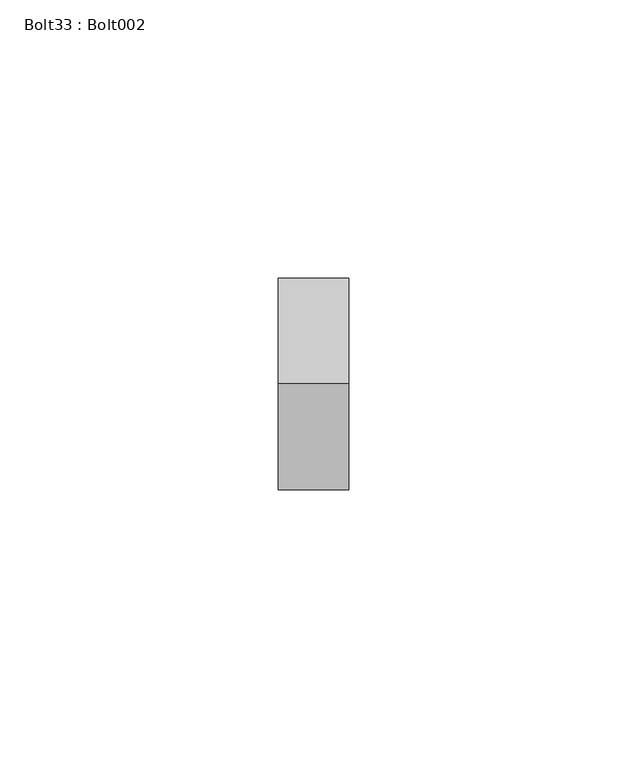
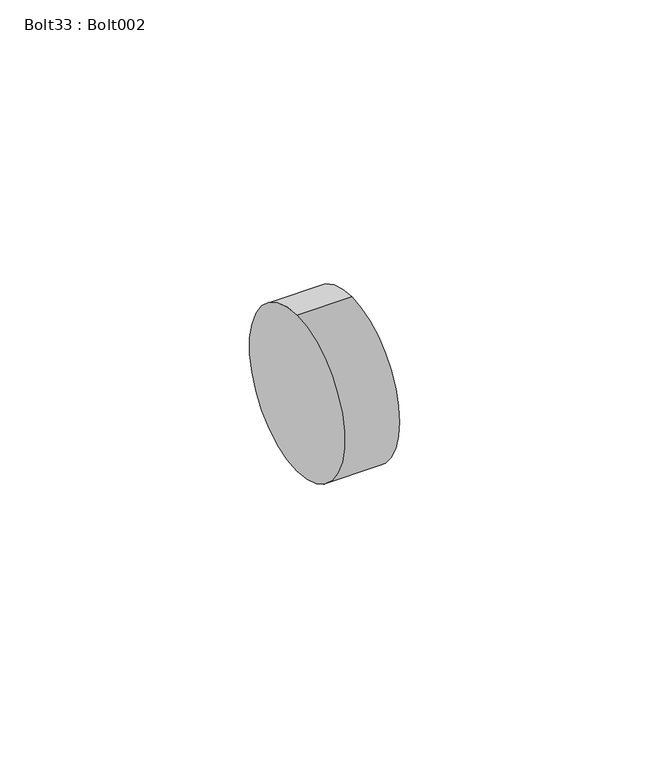
"""IFC4 building model written with IfcOpenShell, lengths in millimetres: proxy geometry, Bolt33 : Bolt002."""

import ifcopenshell
import ifcopenshell.guid

model = None  # the IFC model being written
_history = None  # IfcOwnerHistory: only IFC2X3 demands one
_inside = {}  # id of a spatial element -> (the spatial element, [elements in it])
_under = {}  # id of a project, library or spatial element -> (it, [spatial elements below it])
_declared = {}  # id of a project -> (the project, [libraries it declares])
_typed = {}  # id of a type object -> (the type object, [elements of that type])
_made_of = {}  # id of a material, layer set ... -> (it, [elements and type objects made of it])


def new_model(schema):
    """Start an empty IFC model of exactly this schema.

    Asked for "IFC4X3", IfcOpenShell would pick the latest addendum, in which some entities
    have other attributes; the version numbers below select the first issue.
    IFC2X3 requires an IfcOwnerHistory on every rooted entity: one is made here for all.
    """
    global model, _history
    if schema == "IFC4X3":
        model = ifcopenshell.file(schema_version=(4, 3, 0, 0))
    else:
        model = ifcopenshell.file(schema=schema)
    _inside.clear()
    _under.clear()
    _declared.clear()
    _typed.clear()
    _made_of.clear()
    _history = None
    if model.schema == "IFC2X3":
        org = make("IfcOrganization", Name="unknown")
        user = make(
            "IfcPersonAndOrganization",
            ThePerson=make("IfcPerson", FamilyName="unknown"),
            TheOrganization=org,
        )
        app = make(
            "IfcApplication",
            ApplicationDeveloper=org,
            Version="unknown",
            ApplicationFullName="unknown",
            ApplicationIdentifier="unknown",
        )
        _history = make(
            "IfcOwnerHistory",
            OwningUser=user,
            OwningApplication=app,
            ChangeAction="ADDED",
            CreationDate=0,
        )
    return model


def make(cls, **values):
    """One entity of the class cls with the attributes given. An attribute that is None is left unset."""
    return model.create_entity(
        cls, **{name: value for name, value in values.items() if value is not None}
    )


def rooted(cls, **values):
    """An entity with a GlobalId (a new one), such as an element, a storey or a relation."""
    return make(cls, GlobalId=ifcopenshell.guid.new(), OwnerHistory=_history, **values)


def si_unit(unit_type, name, prefix=None):
    """IfcSIUnit, for example si_unit("LENGTHUNIT", "METRE", prefix="MILLI")."""
    return make("IfcSIUnit", UnitType=unit_type, Prefix=prefix, Name=name)


def assignment(units):
    """IfcUnitAssignment: the units of a project."""
    return None if units is None else make("IfcUnitAssignment", Units=units)


def point(xyz):
    """IfcCartesianPoint."""
    return None if xyz is None else make("IfcCartesianPoint", Coordinates=xyz)


def direction(xyz):
    """IfcDirection."""
    return None if xyz is None else make("IfcDirection", DirectionRatios=xyz)


def frame(location, z_axis=None, x_axis=None):
    """IfcAxis2Placement3D, a coordinate frame: its origin and axes. An axis left out is left unset."""
    return make(
        "IfcAxis2Placement3D",
        Location=point(location),
        Axis=direction(z_axis),
        RefDirection=direction(x_axis),
    )


def frame_2d(location, x_axis=None):
    """IfcAxis2Placement2D, a coordinate frame in the plane: its origin and x axis."""
    return make(
        "IfcAxis2Placement2D", Location=point(location), RefDirection=direction(x_axis)
    )


def origin():
    """The frame at (0, 0, 0) with its axes left unset."""
    return frame((0.0, 0.0, 0.0))


def place(relative_to, where):
    """IfcLocalPlacement: puts the frame where relative to a parent placement (None: the world)."""
    return make(
        "IfcLocalPlacement", PlacementRelTo=relative_to, RelativePlacement=where
    )


def context(
    kind, dimensions, precision=None, world=None, true_north=None, identifier=None
):
    """IfcGeometricRepresentationContext, for example the 3D "Model" context."""
    return make(
        "IfcGeometricRepresentationContext",
        ContextIdentifier=identifier,
        ContextType=kind,
        CoordinateSpaceDimension=dimensions,
        Precision=precision,
        WorldCoordinateSystem=world,
        TrueNorth=true_north,
    )


def project(units=None, contexts=None):
    """IfcProject with its units and contexts."""
    return rooted(
        "IfcProject",
        Name="project",
        RepresentationContexts=contexts,
        UnitsInContext=assignment(units),
    )


def spatial(cls, under=None, at=None, **own):
    """A site, building, storey or space (cls), placed at a placement, below another one or the project."""
    s = rooted(cls, ObjectPlacement=at, **own)
    if under is not None:
        _under.setdefault(under.id(), (under, []))[1].append(s)
    return s


def circle_curve(where, radius):
    """IfcCircle in the frame where."""
    return make("IfcCircle", Position=where, Radius=radius)


def trimmed(basis, trim1, trim2, sense, master):
    """IfcTrimmedCurve: the piece of a basis curve between two trims."""
    return make(
        "IfcTrimmedCurve",
        BasisCurve=basis,
        Trim1=trim1,
        Trim2=trim2,
        SenseAgreement=sense,
        MasterRepresentation=master,
    )


def segment(curve, same_sense, transition):
    """IfcCompositeCurveSegment."""
    return make(
        "IfcCompositeCurveSegment",
        Transition=transition,
        SameSense=same_sense,
        ParentCurve=curve,
    )


def composite_curve(segments, self_intersect=None):
    """IfcCompositeCurve: segments joined end to end."""
    return make("IfcCompositeCurve", Segments=segments, SelfIntersect=self_intersect)


def outline(outer, holes=None, kind="AREA"):
    """IfcArbitraryClosedProfileDef: a profile drawn as a closed curve; with holes, ...WithVoids."""
    if holes is None:
        return make("IfcArbitraryClosedProfileDef", ProfileType=kind, OuterCurve=outer)
    return make(
        "IfcArbitraryProfileDefWithVoids",
        ProfileType=kind,
        OuterCurve=outer,
        InnerCurves=holes,
    )


def extrude(swept, where, along, depth):
    """IfcExtrudedAreaSolid: the profile swept, set in the frame where, extruded along a direction by depth."""
    return make(
        "IfcExtrudedAreaSolid",
        SweptArea=swept,
        Position=where,
        ExtrudedDirection=direction(along),
        Depth=depth,
    )


def shape(context_of_items, identifier, shape_type, items):
    """IfcShapeRepresentation: the items that make up one representation, for example the "Body"."""
    return make(
        "IfcShapeRepresentation",
        ContextOfItems=context_of_items,
        RepresentationIdentifier=identifier,
        RepresentationType=shape_type,
        Items=items,
    )


def source(mapping_origin, context_of_items, identifier, shape_type, items):
    """IfcRepresentationMap: a shape defined once, which mapped items show again and again."""
    return make(
        "IfcRepresentationMap",
        MappingOrigin=mapping_origin,
        MappedRepresentation=shape(context_of_items, identifier, shape_type, items),
    )


def transform(
    local_origin,
    x_axis=None,
    y_axis=None,
    z_axis=None,
    scale=None,
    scale2=None,
    scale3=None,
    uniform=True,
):
    """IfcCartesianTransformationOperator3D, or its non-uniform kind. x_axis, y_axis, z_axis: its Axis1, 2, 3."""
    if uniform:
        return make(
            "IfcCartesianTransformationOperator3D",
            Axis1=direction(x_axis),
            Axis2=direction(y_axis),
            LocalOrigin=point(local_origin),
            Scale=scale,
            Axis3=direction(z_axis),
        )
    return make(
        "IfcCartesianTransformationOperator3DnonUniform",
        Axis1=direction(x_axis),
        Axis2=direction(y_axis),
        LocalOrigin=point(local_origin),
        Scale=scale,
        Axis3=direction(z_axis),
        Scale2=scale2,
        Scale3=scale3,
    )


def mapped(mapping_source, mapping_target):
    """IfcMappedItem: shows the shape of a source again, moved by a transform."""
    return make(
        "IfcMappedItem", MappingSource=mapping_source, MappingTarget=mapping_target
    )


def made_of(thing, what):
    """Note that an element or type object is made of a material, layer set ...; save() writes the relation."""
    if what is not None:
        _made_of.setdefault(what.id(), (what, []))[1].append(thing)
    return thing


def element(
    cls,
    number,
    at=None,
    inside=None,
    cuts=None,
    type_object=None,
    material=None,
    context=None,
    identifier="Body",
    shape_type=None,
    held_by="IfcProductDefinitionShape",
    body=None,
    shapes=None,
    **own,
):
    """One element of the class cls, such as IfcWall. Its Tag is "e" and its number.

    at: its placement. inside: the storey or other place that contains it. cuts: it is an
    opening in that element (IfcRelVoidsElement). A single representation is given by context,
    identifier, shape_type and body (its items); several are given by shapes. held_by: the class
    of the entity that holds the representations. save() writes the other relations.
    """
    e = rooted(cls, Tag="e%d" % number, ObjectPlacement=at, **own)
    if body is not None:
        shapes = [shape(context, identifier, shape_type, body)]
    if shapes is not None:
        e.Representation = make(held_by, Representations=shapes)
    if inside is not None:
        _inside.setdefault(inside.id(), (inside, []))[1].append(e)
    if cuts is not None:
        rooted(
            "IfcRelVoidsElement", RelatingBuildingElement=cuts, RelatedOpeningElement=e
        )
    if type_object is not None:
        _typed.setdefault(type_object.id(), (type_object, []))[1].append(e)
    return made_of(e, material)


def aggregate(whole, parts):
    """IfcRelAggregates: a whole, such as a stair, and the parts it consists of."""
    return rooted("IfcRelAggregates", RelatingObject=whole, RelatedObjects=parts)


def save(model, path):
    """Write the relations noted so far, then the file.

    IfcRelAggregates (storeys below a building ...), IfcRelContainedInSpatialStructure (elements
    in a storey), IfcRelDefinesByType, IfcRelAssociatesMaterial and IfcRelDeclares: one each for
    every whole, place, type object, material and project.
    """
    for whole, parts in _under.values():
        aggregate(whole, parts)
    for where, things in _inside.values():
        rooted(
            "IfcRelContainedInSpatialStructure",
            RelatedElements=things,
            RelatingStructure=where,
        )
    for kind, things in _typed.values():
        rooted("IfcRelDefinesByType", RelatedObjects=things, RelatingType=kind)
    for what, things in _made_of.values():
        rooted("IfcRelAssociatesMaterial", RelatedObjects=things, RelatingMaterial=what)
    for by, libraries in _declared.values():
        rooted("IfcRelDeclares", RelatingContext=by, RelatedDefinitions=libraries)
    model.write(path)


def bolt33_bolt002_dc929be4(model_context):
    return source(origin(), model_context, "Body", "SweptSolid", [
        extrude(outline(composite_curve([segment(trimmed(circle_curve(frame_2d((1896.5882072, 40070.0545241)), 19.05), [point((1896.5882072, 40051.0045241))], [point((1896.5882072, 40089.1045241))], False, "CARTESIAN"), True, "CONTINUOUS"), segment(trimmed(circle_curve(frame_2d((1896.5882072, 40070.0545241)), 19.05), [point((1896.5882072, 40089.1045241))], [point((1896.5882072, 40051.0045241))], False, "CARTESIAN"), True, "CONTINUOUS")], self_intersect=False)), frame((10268.2640809, 0.0, 0.0), z_axis=(1.0, 0.0, 0.0), x_axis=(0.0, 1.0, 0.0)), (0.0, 0.0, 1.0), 12.7),
    ])


if __name__ == "__main__":
    model = new_model("IFC4")
    model_context = context("Model", 3, world=origin())
    ifc_project = project(units=[si_unit("LENGTHUNIT", "METRE", prefix="MILLI")], contexts=[model_context])
    site = spatial("IfcSite", under=ifc_project)
    building = spatial("IfcBuilding", under=site)
    placement = place(None, origin())
    bolt33_bolt002_shape = bolt33_bolt002_dc929be4(model_context)
    element("IfcBuildingElementProxy", 1, Name="Bolt33 : Bolt002", ObjectType="Bolt33 : Bolt002", at=placement, inside=building, context=model_context, shape_type="MappedRepresentation", body=[
        mapped(bolt33_bolt002_shape, transform((0.0, 0.0, 0.0), x_axis=(1.0, 0.0, 0.0), y_axis=(0.0, 1.0, 0.0), z_axis=(0.0, 0.0, 1.0))),
    ])
    save(model, "model.ifc")

# Revit data of these elements
# Type "Bolt33 : Bolt002"
#   NameOverride = "Bolt002"
# Element 1 (IfcBuildingElementProxy, "Bolt33 : Bolt002")
#   Materials on its faces: "STEEL ANGLE AND ANCHOR BOLT (SEE STRUCT. DWGS)"
# Materials
#   "STEEL ANGLE AND ANCHOR BOLT (SEE STRUCT. DWGS)": class "Unassigned", colour RGB 128 128 128, transparency 0, Cost = 0
